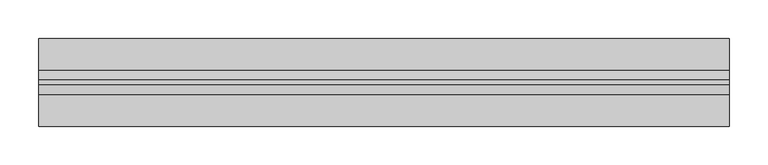
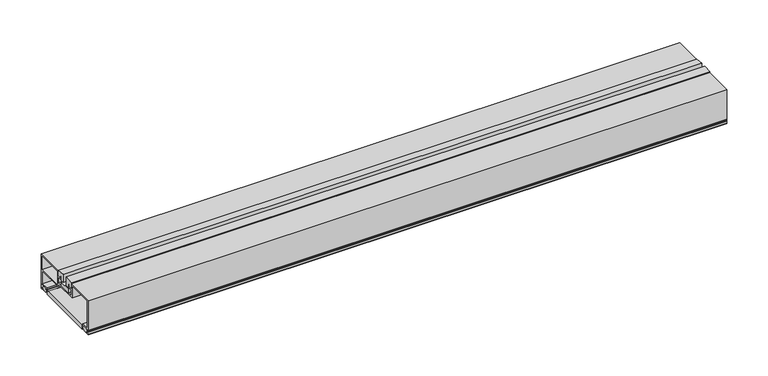
"""IFC4 building model written with IfcOpenShell, lengths in millimetres: proxy geometry, Generic Models 3:Generic Models 1:2:Generic Models 1:2 : Generic Models 3:Generic Models 1:300625:328150:Generic Models 1:2:Generic Models 1:2 : Generic Models 3:Generic Models 1:300625:328150 : Generic Models 3:Generic Models 1:2:Generic Models 1:2 : Generic Models 3:Generic Models 1:300625:328150:3 : Generic Models 3:Generic Models 1:2:Generic Models 1:2 : Generic Models 3:Generic Models 1:300625:328150:Generic Models 1:2:Generic Models 1:2 : Generic Models 3:Generic Models 1:300625:328150 : Generic Models 3:Generic Models 1:2:Generic Models 1:2 : Generic Models 3:Generic Models 1:300625:328150:300962."""

import ifcopenshell
import ifcopenshell.guid

model = None  # the IFC model being written
_history = None  # IfcOwnerHistory: only IFC2X3 demands one
_inside = {}  # id of a spatial element -> (the spatial element, [elements in it])
_under = {}  # id of a project, library or spatial element -> (it, [spatial elements below it])
_declared = {}  # id of a project -> (the project, [libraries it declares])
_typed = {}  # id of a type object -> (the type object, [elements of that type])
_made_of = {}  # id of a material, layer set ... -> (it, [elements and type objects made of it])


def new_model(schema):
    """Start an empty IFC model of exactly this schema.

    Asked for "IFC4X3", IfcOpenShell would pick the latest addendum, in which some entities
    have other attributes; the version numbers below select the first issue.
    IFC2X3 requires an IfcOwnerHistory on every rooted entity: one is made here for all.
    """
    global model, _history
    if schema == "IFC4X3":
        model = ifcopenshell.file(schema_version=(4, 3, 0, 0))
    else:
        model = ifcopenshell.file(schema=schema)
    _inside.clear()
    _under.clear()
    _declared.clear()
    _typed.clear()
    _made_of.clear()
    _history = None
    if model.schema == "IFC2X3":
        org = make("IfcOrganization", Name="unknown")
        user = make(
            "IfcPersonAndOrganization",
            ThePerson=make("IfcPerson", FamilyName="unknown"),
            TheOrganization=org,
        )
        app = make(
            "IfcApplication",
            ApplicationDeveloper=org,
            Version="unknown",
            ApplicationFullName="unknown",
            ApplicationIdentifier="unknown",
        )
        _history = make(
            "IfcOwnerHistory",
            OwningUser=user,
            OwningApplication=app,
            ChangeAction="ADDED",
            CreationDate=0,
        )
    return model


def make(cls, **values):
    """One entity of the class cls with the attributes given. An attribute that is None is left unset."""
    return model.create_entity(
        cls, **{name: value for name, value in values.items() if value is not None}
    )


def rooted(cls, **values):
    """An entity with a GlobalId (a new one), such as an element, a storey or a relation."""
    return make(cls, GlobalId=ifcopenshell.guid.new(), OwnerHistory=_history, **values)


def si_unit(unit_type, name, prefix=None):
    """IfcSIUnit, for example si_unit("LENGTHUNIT", "METRE", prefix="MILLI")."""
    return make("IfcSIUnit", UnitType=unit_type, Prefix=prefix, Name=name)


def assignment(units):
    """IfcUnitAssignment: the units of a project."""
    return None if units is None else make("IfcUnitAssignment", Units=units)


def point(xyz):
    """IfcCartesianPoint."""
    return None if xyz is None else make("IfcCartesianPoint", Coordinates=xyz)


def direction(xyz):
    """IfcDirection."""
    return None if xyz is None else make("IfcDirection", DirectionRatios=xyz)


def frame(location, z_axis=None, x_axis=None):
    """IfcAxis2Placement3D, a coordinate frame: its origin and axes. An axis left out is left unset."""
    return make(
        "IfcAxis2Placement3D",
        Location=point(location),
        Axis=direction(z_axis),
        RefDirection=direction(x_axis),
    )


def origin():
    """The frame at (0, 0, 0) with its axes left unset."""
    return frame((0.0, 0.0, 0.0))


def place(relative_to, where):
    """IfcLocalPlacement: puts the frame where relative to a parent placement (None: the world)."""
    return make(
        "IfcLocalPlacement", PlacementRelTo=relative_to, RelativePlacement=where
    )


def context(
    kind, dimensions, precision=None, world=None, true_north=None, identifier=None
):
    """IfcGeometricRepresentationContext, for example the 3D "Model" context."""
    return make(
        "IfcGeometricRepresentationContext",
        ContextIdentifier=identifier,
        ContextType=kind,
        CoordinateSpaceDimension=dimensions,
        Precision=precision,
        WorldCoordinateSystem=world,
        TrueNorth=true_north,
    )


def project(units=None, contexts=None):
    """IfcProject with its units and contexts."""
    return rooted(
        "IfcProject",
        Name="project",
        RepresentationContexts=contexts,
        UnitsInContext=assignment(units),
    )


def spatial(cls, under=None, at=None, **own):
    """A site, building, storey or space (cls), placed at a placement, below another one or the project."""
    s = rooted(cls, ObjectPlacement=at, **own)
    if under is not None:
        _under.setdefault(under.id(), (under, []))[1].append(s)
    return s


def polyline(points):
    """IfcPolyline through the points."""
    return make("IfcPolyline", Points=[point(p) for p in points])


def outline(outer, holes=None, kind="AREA"):
    """IfcArbitraryClosedProfileDef: a profile drawn as a closed curve; with holes, ...WithVoids."""
    if holes is None:
        return make("IfcArbitraryClosedProfileDef", ProfileType=kind, OuterCurve=outer)
    return make(
        "IfcArbitraryProfileDefWithVoids",
        ProfileType=kind,
        OuterCurve=outer,
        InnerCurves=holes,
    )


def extrude(swept, where, along, depth):
    """IfcExtrudedAreaSolid: the profile swept, set in the frame where, extruded along a direction by depth."""
    return make(
        "IfcExtrudedAreaSolid",
        SweptArea=swept,
        Position=where,
        ExtrudedDirection=direction(along),
        Depth=depth,
    )


def shape(context_of_items, identifier, shape_type, items):
    """IfcShapeRepresentation: the items that make up one representation, for example the "Body"."""
    return make(
        "IfcShapeRepresentation",
        ContextOfItems=context_of_items,
        RepresentationIdentifier=identifier,
        RepresentationType=shape_type,
        Items=items,
    )


def source(mapping_origin, context_of_items, identifier, shape_type, items):
    """IfcRepresentationMap: a shape defined once, which mapped items show again and again."""
    return make(
        "IfcRepresentationMap",
        MappingOrigin=mapping_origin,
        MappedRepresentation=shape(context_of_items, identifier, shape_type, items),
    )


def transform(
    local_origin,
    x_axis=None,
    y_axis=None,
    z_axis=None,
    scale=None,
    scale2=None,
    scale3=None,
    uniform=True,
):
    """IfcCartesianTransformationOperator3D, or its non-uniform kind. x_axis, y_axis, z_axis: its Axis1, 2, 3."""
    if uniform:
        return make(
            "IfcCartesianTransformationOperator3D",
            Axis1=direction(x_axis),
            Axis2=direction(y_axis),
            LocalOrigin=point(local_origin),
            Scale=scale,
            Axis3=direction(z_axis),
        )
    return make(
        "IfcCartesianTransformationOperator3DnonUniform",
        Axis1=direction(x_axis),
        Axis2=direction(y_axis),
        LocalOrigin=point(local_origin),
        Scale=scale,
        Axis3=direction(z_axis),
        Scale2=scale2,
        Scale3=scale3,
    )


def mapped(mapping_source, mapping_target):
    """IfcMappedItem: shows the shape of a source again, moved by a transform."""
    return make(
        "IfcMappedItem", MappingSource=mapping_source, MappingTarget=mapping_target
    )


def made_of(thing, what):
    """Note that an element or type object is made of a material, layer set ...; save() writes the relation."""
    if what is not None:
        _made_of.setdefault(what.id(), (what, []))[1].append(thing)
    return thing


def element(
    cls,
    number,
    at=None,
    inside=None,
    cuts=None,
    type_object=None,
    material=None,
    context=None,
    identifier="Body",
    shape_type=None,
    held_by="IfcProductDefinitionShape",
    body=None,
    shapes=None,
    **own,
):
    """One element of the class cls, such as IfcWall. Its Tag is "e" and its number.

    at: its placement. inside: the storey or other place that contains it. cuts: it is an
    opening in that element (IfcRelVoidsElement). A single representation is given by context,
    identifier, shape_type and body (its items); several are given by shapes. held_by: the class
    of the entity that holds the representations. save() writes the other relations.
    """
    e = rooted(cls, Tag="e%d" % number, ObjectPlacement=at, **own)
    if body is not None:
        shapes = [shape(context, identifier, shape_type, body)]
    if shapes is not None:
        e.Representation = make(held_by, Representations=shapes)
    if inside is not None:
        _inside.setdefault(inside.id(), (inside, []))[1].append(e)
    if cuts is not None:
        rooted(
            "IfcRelVoidsElement", RelatingBuildingElement=cuts, RelatedOpeningElement=e
        )
    if type_object is not None:
        _typed.setdefault(type_object.id(), (type_object, []))[1].append(e)
    return made_of(e, material)


def aggregate(whole, parts):
    """IfcRelAggregates: a whole, such as a stair, and the parts it consists of."""
    return rooted("IfcRelAggregates", RelatingObject=whole, RelatedObjects=parts)


def save(model, path):
    """Write the relations noted so far, then the file.

    IfcRelAggregates (storeys below a building ...), IfcRelContainedInSpatialStructure (elements
    in a storey), IfcRelDefinesByType, IfcRelAssociatesMaterial and IfcRelDeclares: one each for
    every whole, place, type object, material and project.
    """
    for whole, parts in _under.values():
        aggregate(whole, parts)
    for where, things in _inside.values():
        rooted(
            "IfcRelContainedInSpatialStructure",
            RelatedElements=things,
            RelatingStructure=where,
        )
    for kind, things in _typed.values():
        rooted("IfcRelDefinesByType", RelatedObjects=things, RelatingType=kind)
    for what, things in _made_of.values():
        rooted("IfcRelAssociatesMaterial", RelatedObjects=things, RelatingMaterial=what)
    for by, libraries in _declared.values():
        rooted("IfcRelDeclares", RelatingContext=by, RelatedDefinitions=libraries)
    model.write(path)


def generic_models_21ac7cc4(model_context):
    return source(origin(), model_context, "Body", "SweptSolid", [
        extrude(outline(polyline([(-568050.8100714, 46.8872108), (-568050.8100714, 41.1736702), (-568055.5641272, 41.1736702), (-568055.5641272, 53.2439273), (-568043.6663214, 51.7830605), (-568043.6663214, 43.9433511), (-568047.9643932, 43.9433511), (-568047.9643932, 46.8872108), (-568050.8100714, 46.8872108)])), frame((592836.3867242, 0.0, 0.0), z_axis=(1.0, 0.0, 0.0), x_axis=(0.0, 1.0, 0.0)), (0.0, 0.0, 1.0), 895.35),
        extrude(outline(polyline([(593731.7367242, -568016.9406051), (593731.7367242, -568102.342163), (592836.3867242, -568102.342163), (592836.3867242, -568016.9406051), (593731.7367242, -568016.9406051)])), frame((0.0, 0.0, 0.0018625), z_axis=(0.0, 0.0, 1.0), x_axis=(1.0, 0.0, 0.0)), (0.0, 0.0, 1.0), 6.35),
        extrude(outline(polyline([(-568002.371855, 5.3860992), (-568002.6855411, 3.1768625), (-568002.371855, 0.9676257), (-568001.9944464, 0.0018625), (-568007.8625385, 0.0018625), (-568007.0022575, 0.38818), (-568005.6926824, 1.4716655), (-568005.0923289, 2.8219132), (-568005.2951168, 4.2276895), (-568006.2693218, 5.4690736), (-568007.8625385, 6.3518625), (-568001.9944464, 6.3518625), (-568002.371855, 5.3860992)])), frame((592836.3867242, 0.0, 0.0), z_axis=(1.0, 0.0, 0.0), x_axis=(0.0, 1.0, 0.0)), (0.0, 0.0, 1.0), 895.35),
        extrude(outline(polyline([(-568005.9353019, 1.7992816), (-568007.2567959, 0.6945475), (-568009.1664101, 0.0814663), (-568010.2261661, 0.0018625), (-568011.285922, 0.0814663), (-568013.1955363, 0.6945475), (-568014.5170303, 1.7992816), (-568014.9886661, 3.1768625), (-568014.5170303, 4.5544433), (-568013.1955363, 5.6591774), (-568011.285922, 6.2722586), (-568010.2261661, 6.3518625), (-568009.1664101, 6.2722586), (-568007.2567959, 5.6591774), (-568005.9353019, 4.5544433), (-568005.4636661, 3.1768625), (-568005.9353019, 1.7992816)])), frame((592836.3867242, 0.0, 0.0), z_axis=(1.0, 0.0, 0.0), x_axis=(0.0, 1.0, 0.0)), (0.0, 0.0, 1.0), 895.35),
        extrude(outline(polyline([(-568107.0029708, 0.0814663), (-568108.0627267, 0.0018625), (-568109.1224826, 0.0814663), (-568111.0320969, 0.6945475), (-568112.3535909, 1.7992816), (-568112.8252267, 3.1768625), (-568112.3535909, 4.5544433), (-568111.0320969, 5.6591774), (-568109.1224826, 6.2722586), (-568108.0627267, 6.3518625), (-568107.0029708, 6.2722586), (-568105.0933565, 5.6591774), (-568103.7718625, 4.5544433), (-568103.3002267, 3.1768625), (-568103.7718625, 1.7992816), (-568105.0933565, 0.6945475), (-568107.0029708, 0.0814663)])), frame((592836.3867242, 0.0, 0.0), z_axis=(1.0, 0.0, 0.0), x_axis=(0.0, 1.0, 0.0)), (0.0, 0.0, 1.0), 895.35),
        extrude(outline(polyline([(-568110.4263543, 0.0018625), (-568116.2944464, 0.0018625), (-568115.9170378, 0.9676257), (-568115.6033517, 3.1768625), (-568115.9170378, 5.3860992), (-568116.2944464, 6.3518625), (-568110.4263543, 6.3518625), (-568112.019571, 5.4690736), (-568112.993776, 4.2276895), (-568113.1965639, 2.8219132), (-568112.5962104, 1.4716655), (-568111.2866352, 0.38818), (-568110.4263543, 0.0018625)])), frame((592836.3867242, 0.0, 0.0), z_axis=(1.0, 0.0, 0.0), x_axis=(0.0, 1.0, 0.0)), (0.0, 0.0, 1.0), 895.35),
        extrude(outline(polyline([(593731.7367242, -568050.8100714), (593731.7367242, -568067.4788214), (592836.3867242, -568067.4788214), (592836.3867242, -568050.8100714), (593731.7367242, -568050.8100714)])), frame((0.0, 0.0, 32.9494693), z_axis=(0.0, 0.0, 1.0), x_axis=(1.0, 0.0, 0.0)), (0.0, 0.0, 1.0), 5.5626),
        extrude(outline(polyline([(-568067.4788214, 46.8872108), (-568070.3244996, 46.8872108), (-568070.3244996, 43.9433511), (-568074.6225714, 43.9433511), (-568074.6225714, 51.7830605), (-568062.7247655, 53.2439273), (-568062.7247655, 41.1736702), (-568067.4788214, 41.1736702), (-568067.4788214, 46.8872108)])), frame((592836.3867242, 0.0, 0.0), z_axis=(1.0, 0.0, 0.0), x_axis=(0.0, 1.0, 0.0)), (0.0, 0.0, 1.0), 895.35),
        extrude(outline(polyline([(-568116.2944464, 6.35), (-568116.2944464, 50.7662234), (-568074.9780601, 50.7662234), (-568074.9780601, 43.5464761), (-568069.8862383, 43.5464761), (-568069.8862383, 46.4903358), (-568067.8343101, 46.4903358), (-568067.8343101, 41.5705452), (-568074.9780601, 41.5705452), (-568074.9780601, 32.9494693), (-568043.3108327, 32.9494693), (-568043.3108327, 41.5705452), (-568050.4545827, 41.5705452), (-568050.4545827, 46.4903358), (-568048.4026545, 46.4903358), (-568048.4026545, 43.5464761), (-568043.3108327, 43.5464761), (-568043.3108327, 50.7662234), (-568001.9944464, 50.7662234), (-568001.9944464, 6.35), (-568015.0815775, 6.35), (-568015.0815775, 8.2499335), (-568004.5023586, 8.2499335), (-568004.5023586, 27.4630693), (-568043.3108327, 27.4630693), (-568043.3108327, 31.0495358), (-568076.8779936, 31.0495358), (-568076.8779936, 48.8662899), (-568113.7865342, 48.8662899), (-568113.7865342, 8.2499335), (-568103.2073153, 8.2499335), (-568103.2073153, 6.35), (-568116.2944464, 6.35)]), holes=[polyline([(-568041.4108992, 29.3630028), (-568004.5023586, 29.3630028), (-568004.5023586, 48.8662899), (-568041.4108992, 48.8662899), (-568041.4108992, 29.3630028)])]), frame((592836.3867242, 0.0, 0.0), z_axis=(1.0, 0.0, 0.0), x_axis=(0.0, 1.0, 0.0)), (0.0, 0.0, 1.0), 895.35),
    ])


if __name__ == "__main__":
    model = new_model("IFC4")
    model_context = context("Model", 3, world=origin())
    ifc_project = project(units=[si_unit("LENGTHUNIT", "METRE", prefix="MILLI")], contexts=[model_context])
    site = spatial("IfcSite", under=ifc_project)
    building = spatial("IfcBuilding", under=site)
    placement = place(None, origin())
    generic_models_shape = generic_models_21ac7cc4(model_context)
    element("IfcBuildingElementProxy", 1, Name="Generic Models 3:Generic Models 1:2:Generic Models 1:2 : Generic Models 3:Generic Models 1:300625:328150:Generic Models 1:2:Generic Models 1:2 : Generic Models 3:Generic Models 1:300625:328150 : Generic Models 3:Generic Models 1:2:Generic Models 1:2 : Generic Models 3:Generic Models 1:300625:328150:3 : Generic Models 3:Generic Models 1:2:Generic Models 1:2 : Generic Models 3:Generic Models 1:300625:328150:Generic Models 1:2:Generic Models 1:2 : Generic Models 3:Generic Models 1:300625:328150 : Generic Models 3:Generic Models 1:2:Generic Models 1:2 : Generic Models 3:Generic Models 1:300625:328150:300962", ObjectType="Generic Models 3:Generic Models 1:2:Generic Models 1:2 : Generic Models 3:Generic Models 1:300625:328150:Generic Models 1:2:Generic Models 1:2 : Generic Models 3:Generic Models 1:300625:328150 : Generic Models 3:Generic Models 1:2:Generic Models 1:2 : Generic Models 3:Generic Models 1:300625:328150:3 : Generic Models 3:Generic Models 1:2:Generic Models 1:2 : Generic Models 3:Generic Models 1:300625:328150:Generic Models 1:2:Generic Models 1:2 : Generic Models 3:Generic Models 1:300625:328150 : Generic Models 3:Generic Models 1:2:Generic Models 1:2 : Generic Models 3:Generic Models 1:300625:328150:300962", at=placement, inside=building, context=model_context, shape_type="MappedRepresentation", body=[
        mapped(generic_models_shape, transform((0.0, 0.0, 0.0), x_axis=(1.0, 0.0, 0.0), y_axis=(0.0, 1.0, 0.0), z_axis=(0.0, 0.0, 1.0))),
    ])
    save(model, "model.ifc")

# Revit data of these elements
# Type "Generic Models 3:Generic Models 1:2:Generic Models 1:2 : Generic Models 3:Generic Models 1:300625:328150:Generic Models 1:2:Generic Models 1:2 : Generic Models 3:Generic Models 1:300625:328150 : Generic Models 3:Generic Models 1:2:Generic Models 1:2 : Generic Models 3:Generic Models 1:300625:328150:3 : Generic Models 3:Generic Models 1:2:Generic Models 1:2 : Generic Models 3:Generic Models 1:300625:328150:Generic Models 1:2:Generic Models 1:2 : Generic Models 3:Generic Models 1:300625:328150 : Generic Models 3:Generic Models 1:2:Generic Models 1:2 : Generic Models 3:Generic Models 1:300625:328150:300962"
#   NameOverride = "Generic Models 3:Generic Models 1:2:Generic Models 1:2 : Generic Models 3:Generic Models 1:300625:328150:Generic Models 1:2:Generic Models 1:2 : Generic Models 3:Generic Models 1:300625:328150 : Generic Models 3:Generic Models 1:2:Generic Models 1:2 : Generic Models 3:Generic Models 1:300625:328150:300962"
#   ObjectTypeOverride = "Generic Models 1:2:Generic Models 1:2 : Generic Models 3:Generic Models 1:300625:328150 : Generic Models 3:Generic Models 1:2:Generic Models 1:2 : Generic Models 3:Generic Models 1:300625:328150"
#   Reference = "Generic Models 1"
#   Tag = "300962"
# Element 1 (IfcBuildingElementProxy, "Generic Models 3:Generic Models 1:2:Generic Models 1:2 : Generic Models 3:Generic Models 1:300625:328150:Generic Models 1:2:Generic Models 1:2 : Generic Models 3:Generic Models 1:300625:328150 : Generic Models 3:Generic Models 1:2:Generic Models 1:2 : Generic Models 3:Generic Models 1:300625:328150:3 : Generic Models 3:Generic Models 1:2:Generic Models 1:2 : Generic Models 3:Generic Models 1:300625:328150:Generic Models 1:2:Generic Models 1:2 : Generic Models 3:Generic Models 1:300625:328150 : Generic Models 3:Generic Models 1:2:Generic Models 1:2 : Generic Models 3:Generic Models 1:300625:328150:300962")
#   Materials on its faces: "SEALANT & BACKER ROD", "INTERIOR GRADE ALUMINUM STOREFRONT W/ SINGLE GLAZING", "Compression Gasket_1", "Shim_1"
# Materials
#   "SEALANT & BACKER ROD": class "Unassigned", colour RGB 120 120 120, transparency 0, Cost = 0
#   "INTERIOR GRADE ALUMINUM STOREFRONT W/ SINGLE GLAZING": class "Unassigned", colour RGB 244 244 244, transparency 0, Cost = 0
#   "Compression Gasket_1": class "Unassigned", colour RGB 178 178 178, transparency 0
#   "Shim_1": class "Unassigned", colour RGB 218 218 218, transparency 0
